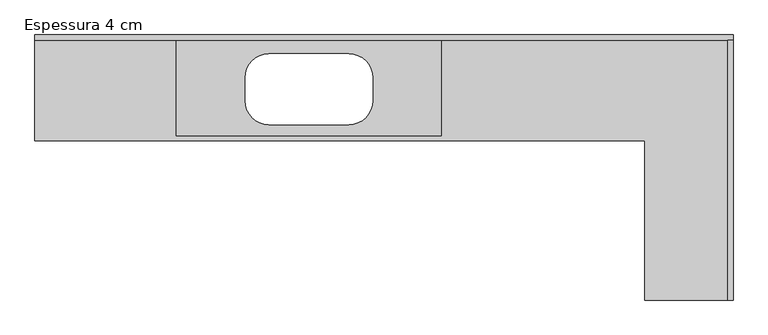
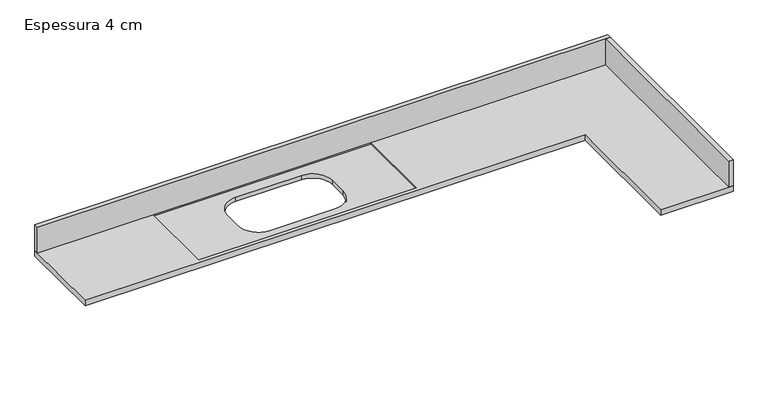
"""IFC4 building model written with IfcOpenShell, lengths in millimetres: furniture geometry, CC_BANCADA-COZINHA_EM-L_CUBA-DUPLA : Espessura 4 cm."""

import ifcopenshell
import ifcopenshell.guid

model = None  # the IFC model being written
_history = None  # IfcOwnerHistory: only IFC2X3 demands one
_inside = {}  # id of a spatial element -> (the spatial element, [elements in it])
_under = {}  # id of a project, library or spatial element -> (it, [spatial elements below it])
_declared = {}  # id of a project -> (the project, [libraries it declares])
_typed = {}  # id of a type object -> (the type object, [elements of that type])
_made_of = {}  # id of a material, layer set ... -> (it, [elements and type objects made of it])


def new_model(schema):
    """Start an empty IFC model of exactly this schema.

    Asked for "IFC4X3", IfcOpenShell would pick the latest addendum, in which some entities
    have other attributes; the version numbers below select the first issue.
    IFC2X3 requires an IfcOwnerHistory on every rooted entity: one is made here for all.
    """
    global model, _history
    if schema == "IFC4X3":
        model = ifcopenshell.file(schema_version=(4, 3, 0, 0))
    else:
        model = ifcopenshell.file(schema=schema)
    _inside.clear()
    _under.clear()
    _declared.clear()
    _typed.clear()
    _made_of.clear()
    _history = None
    if model.schema == "IFC2X3":
        org = make("IfcOrganization", Name="unknown")
        user = make(
            "IfcPersonAndOrganization",
            ThePerson=make("IfcPerson", FamilyName="unknown"),
            TheOrganization=org,
        )
        app = make(
            "IfcApplication",
            ApplicationDeveloper=org,
            Version="unknown",
            ApplicationFullName="unknown",
            ApplicationIdentifier="unknown",
        )
        _history = make(
            "IfcOwnerHistory",
            OwningUser=user,
            OwningApplication=app,
            ChangeAction="ADDED",
            CreationDate=0,
        )
    return model


def make(cls, **values):
    """One entity of the class cls with the attributes given. An attribute that is None is left unset."""
    return model.create_entity(
        cls, **{name: value for name, value in values.items() if value is not None}
    )


def rooted(cls, **values):
    """An entity with a GlobalId (a new one), such as an element, a storey or a relation."""
    return make(cls, GlobalId=ifcopenshell.guid.new(), OwnerHistory=_history, **values)


def si_unit(unit_type, name, prefix=None):
    """IfcSIUnit, for example si_unit("LENGTHUNIT", "METRE", prefix="MILLI")."""
    return make("IfcSIUnit", UnitType=unit_type, Prefix=prefix, Name=name)


def assignment(units):
    """IfcUnitAssignment: the units of a project."""
    return None if units is None else make("IfcUnitAssignment", Units=units)


def point(xyz):
    """IfcCartesianPoint."""
    return None if xyz is None else make("IfcCartesianPoint", Coordinates=xyz)


def direction(xyz):
    """IfcDirection."""
    return None if xyz is None else make("IfcDirection", DirectionRatios=xyz)


def frame(location, z_axis=None, x_axis=None):
    """IfcAxis2Placement3D, a coordinate frame: its origin and axes. An axis left out is left unset."""
    return make(
        "IfcAxis2Placement3D",
        Location=point(location),
        Axis=direction(z_axis),
        RefDirection=direction(x_axis),
    )


def origin():
    """The frame at (0, 0, 0) with its axes left unset."""
    return frame((0.0, 0.0, 0.0))


def place(relative_to, where):
    """IfcLocalPlacement: puts the frame where relative to a parent placement (None: the world)."""
    return make(
        "IfcLocalPlacement", PlacementRelTo=relative_to, RelativePlacement=where
    )


def context(
    kind, dimensions, precision=None, world=None, true_north=None, identifier=None
):
    """IfcGeometricRepresentationContext, for example the 3D "Model" context."""
    return make(
        "IfcGeometricRepresentationContext",
        ContextIdentifier=identifier,
        ContextType=kind,
        CoordinateSpaceDimension=dimensions,
        Precision=precision,
        WorldCoordinateSystem=world,
        TrueNorth=true_north,
    )


def project(units=None, contexts=None):
    """IfcProject with its units and contexts."""
    return rooted(
        "IfcProject",
        Name="project",
        RepresentationContexts=contexts,
        UnitsInContext=assignment(units),
    )


def spatial(cls, under=None, at=None, **own):
    """A site, building, storey or space (cls), placed at a placement, below another one or the project."""
    s = rooted(cls, ObjectPlacement=at, **own)
    if under is not None:
        _under.setdefault(under.id(), (under, []))[1].append(s)
    return s


def polyline(points):
    """IfcPolyline through the points."""
    return make("IfcPolyline", Points=[point(p) for p in points])


def circle_curve(where, radius):
    """IfcCircle in the frame where."""
    return make("IfcCircle", Position=where, Radius=radius)


def outline(outer, holes=None, kind="AREA"):
    """IfcArbitraryClosedProfileDef: a profile drawn as a closed curve; with holes, ...WithVoids."""
    if holes is None:
        return make("IfcArbitraryClosedProfileDef", ProfileType=kind, OuterCurve=outer)
    return make(
        "IfcArbitraryProfileDefWithVoids",
        ProfileType=kind,
        OuterCurve=outer,
        InnerCurves=holes,
    )


def extrude(swept, where, along, depth):
    """IfcExtrudedAreaSolid: the profile swept, set in the frame where, extruded along a direction by depth."""
    return make(
        "IfcExtrudedAreaSolid",
        SweptArea=swept,
        Position=where,
        ExtrudedDirection=direction(along),
        Depth=depth,
    )


def shape(context_of_items, identifier, shape_type, items):
    """IfcShapeRepresentation: the items that make up one representation, for example the "Body"."""
    return make(
        "IfcShapeRepresentation",
        ContextOfItems=context_of_items,
        RepresentationIdentifier=identifier,
        RepresentationType=shape_type,
        Items=items,
    )


def source(mapping_origin, context_of_items, identifier, shape_type, items):
    """IfcRepresentationMap: a shape defined once, which mapped items show again and again."""
    return make(
        "IfcRepresentationMap",
        MappingOrigin=mapping_origin,
        MappedRepresentation=shape(context_of_items, identifier, shape_type, items),
    )


def transform(
    local_origin,
    x_axis=None,
    y_axis=None,
    z_axis=None,
    scale=None,
    scale2=None,
    scale3=None,
    uniform=True,
):
    """IfcCartesianTransformationOperator3D, or its non-uniform kind. x_axis, y_axis, z_axis: its Axis1, 2, 3."""
    if uniform:
        return make(
            "IfcCartesianTransformationOperator3D",
            Axis1=direction(x_axis),
            Axis2=direction(y_axis),
            LocalOrigin=point(local_origin),
            Scale=scale,
            Axis3=direction(z_axis),
        )
    return make(
        "IfcCartesianTransformationOperator3DnonUniform",
        Axis1=direction(x_axis),
        Axis2=direction(y_axis),
        LocalOrigin=point(local_origin),
        Scale=scale,
        Axis3=direction(z_axis),
        Scale2=scale2,
        Scale3=scale3,
    )


def mapped(mapping_source, mapping_target):
    """IfcMappedItem: shows the shape of a source again, moved by a transform."""
    return make(
        "IfcMappedItem", MappingSource=mapping_source, MappingTarget=mapping_target
    )


def made_of(thing, what):
    """Note that an element or type object is made of a material, layer set ...; save() writes the relation."""
    if what is not None:
        _made_of.setdefault(what.id(), (what, []))[1].append(thing)
    return thing


def element(
    cls,
    number,
    at=None,
    inside=None,
    cuts=None,
    type_object=None,
    material=None,
    context=None,
    identifier="Body",
    shape_type=None,
    held_by="IfcProductDefinitionShape",
    body=None,
    shapes=None,
    **own,
):
    """One element of the class cls, such as IfcWall. Its Tag is "e" and its number.

    at: its placement. inside: the storey or other place that contains it. cuts: it is an
    opening in that element (IfcRelVoidsElement). A single representation is given by context,
    identifier, shape_type and body (its items); several are given by shapes. held_by: the class
    of the entity that holds the representations. save() writes the other relations.
    """
    e = rooted(cls, Tag="e%d" % number, ObjectPlacement=at, **own)
    if body is not None:
        shapes = [shape(context, identifier, shape_type, body)]
    if shapes is not None:
        e.Representation = make(held_by, Representations=shapes)
    if inside is not None:
        _inside.setdefault(inside.id(), (inside, []))[1].append(e)
    if cuts is not None:
        rooted(
            "IfcRelVoidsElement", RelatingBuildingElement=cuts, RelatedOpeningElement=e
        )
    if type_object is not None:
        _typed.setdefault(type_object.id(), (type_object, []))[1].append(e)
    return made_of(e, material)


def aggregate(whole, parts):
    """IfcRelAggregates: a whole, such as a stair, and the parts it consists of."""
    return rooted("IfcRelAggregates", RelatingObject=whole, RelatedObjects=parts)


def save(model, path):
    """Write the relations noted so far, then the file.

    IfcRelAggregates (storeys below a building ...), IfcRelContainedInSpatialStructure (elements
    in a storey), IfcRelDefinesByType, IfcRelAssociatesMaterial and IfcRelDeclares: one each for
    every whole, place, type object, material and project.
    """
    for whole, parts in _under.values():
        aggregate(whole, parts)
    for where, things in _inside.values():
        rooted(
            "IfcRelContainedInSpatialStructure",
            RelatedElements=things,
            RelatingStructure=where,
        )
    for kind, things in _typed.values():
        rooted("IfcRelDefinesByType", RelatedObjects=things, RelatingType=kind)
    for what, things in _made_of.values():
        rooted("IfcRelAssociatesMaterial", RelatedObjects=things, RelatingMaterial=what)
    for by, libraries in _declared.values():
        rooted("IfcRelDeclares", RelatingContext=by, RelatedDefinitions=libraries)
    model.write(path)


def plane_surface(at):
    """IfcPlane: the flat surface through the origin of the frame at, square to its z axis."""
    return make("IfcPlane", Position=at)


def revolved_surface(curve, axis_point, axis_direction):
    """IfcSurfaceOfRevolution: the curve turned about the line through axis_point along axis_direction."""
    return make(
        "IfcSurfaceOfRevolution",
        SweptCurve=make("IfcArbitraryOpenProfileDef", ProfileType="CURVE", Curve=curve),
        AxisPosition=make("IfcAxis1Placement", Location=point(axis_point), Axis=direction(axis_direction)),
    )


def advanced_brep(points, edges, surfaces, faces):
    """IfcAdvancedBrep: a solid bounded by faces that lie on surfaces and meet in shared edges.

    An edge is (start, end): straight between two places in points (the first is 0);
    or (start, end, curve); or (start, end, curve, False) where it runs against its curve.
    A face is (place in surfaces, loops), or (place, loops, False) where it looks against
    its surface's normal. A loop lists edges by number (the first is 1), with a minus sign
    where the edge is run from its end to its start. The first loop is the outer one.
    """
    corners = [point(p) for p in points]
    vertices = [make("IfcVertexPoint", VertexGeometry=c) for c in corners]
    made = []
    for start, end, *more in edges:
        made.append(
            make(
                "IfcEdgeCurve",
                EdgeStart=vertices[start],
                EdgeEnd=vertices[end],
                EdgeGeometry=more[0] if more else make("IfcPolyline", Points=[corners[start], corners[end]]),
                SameSense=more[1] if len(more) > 1 else True,
            )
        )
    hull = []
    for where, loops, *sense in faces:
        bounds = []
        for j, loop in enumerate(loops):
            ring = [make("IfcOrientedEdge", EdgeElement=made[abs(k) - 1], Orientation=k > 0) for k in loop]
            bounds.append(
                make(
                    "IfcFaceOuterBound" if j == 0 else "IfcFaceBound",
                    Bound=make("IfcEdgeLoop", EdgeList=ring),
                    Orientation=True,
                )
            )
        hull.append(make("IfcAdvancedFace", Bounds=bounds, FaceSurface=surfaces[where], SameSense=sense[0] if sense else True))
    return make("IfcAdvancedBrep", Outer=make("IfcClosedShell", CfsFaces=hull))


def espessura_4_cm_f782d00c(model_context):
    return source(origin(), model_context, "Body", "SolidModel", [
        extrude(outline(polyline([(-30.0, -30.0), (0.0, -30.0), (0.0, -1500.0), (-30.0, -1500.0), (-30.0, -30.0)])), frame((0.0, 0.0, 900.0), z_axis=(0.0, 0.0, 1.0), x_axis=(1.0, 0.0, 0.0)), (0.0, 0.0, 1.0), 190.0),
        extrude(outline(polyline([(-3950.0, -30.0), (-3950.0, 0.0), (0.0, 0.0), (0.0, -30.0), (-3950.0, -30.0)])), frame((0.0, 0.0, 900.0), z_axis=(0.0, 0.0, 1.0), x_axis=(1.0, 0.0, 0.0)), (0.0, 0.0, 1.0), 190.0),
        advanced_brep(
        [(-500.0, -600.0, 860.0), (-3950.0, -600.0, 860.0), (-3950.0, 0.0, 860.0), (0.0, 0.0, 860.0), (0.0, -1500.0, 860.0), (-500.0, -1500.0, 860.0), (-2626.0, -107.0, 860.0), (-2761.0, -242.0, 860.0), (-2761.0, -372.0, 860.0), (-2626.0, -507.0, 860.0), (-2174.0, -507.0, 860.0), (-2039.0, -372.0, 860.0), (-2039.0, -242.0, 860.0), (-2174.0, -107.0, 860.0), (-500.0, -600.0, 900.0), (-500.0, -1500.0, 900.0), (0.0, -1500.0, 900.0), (0.0, 0.0, 900.0), (-3950.0, 0.0, 900.0), (-3950.0, -600.0, 900.0), (-1650.0, -30.0, 900.0), (-1650.0, -570.0, 900.0), (-3150.0, -570.0, 900.0), (-3150.0, -30.0, 900.0), (-2174.0, -107.0, 890.0), (-2626.0, -107.0, 890.0), (-2039.0, -242.0, 890.0), (-2039.0, -372.0, 890.0), (-2174.0, -507.0, 890.0), (-2626.0, -507.0, 890.0), (-2761.0, -372.0, 890.0), (-2761.0, -242.0, 890.0), (-1650.0, -570.0, 890.0), (-1650.0, -30.0, 890.0), (-3150.0, -30.0, 890.0), (-3150.0, -570.0, 890.0)],
        [
            (0, 1),
            (1, 2),
            (2, 3),
            (3, 4),
            (4, 5),
            (5, 0),
            (6, 7, circle_curve(frame((-2626.0, -242.0, 860.0), z_axis=(0.0, 0.0, 1.0), x_axis=(-1.0, 0.0, 0.0)), 135.0)),
            (7, 8),
            (8, 9, circle_curve(frame((-2626.0, -372.0, 860.0), z_axis=(0.0, 0.0, 1.0), x_axis=(-1.0, 0.0, 0.0)), 135.0)),
            (9, 10),
            (10, 11, circle_curve(frame((-2174.0, -372.0, 860.0), z_axis=(0.0, 0.0, 1.0), x_axis=(-1.0, 0.0, 0.0)), 135.0)),
            (11, 12),
            (12, 13, circle_curve(frame((-2174.0, -242.0, 860.0), z_axis=(0.0, 0.0, 1.0), x_axis=(-1.0, 0.0, 0.0)), 135.0)),
            (13, 6),
            (14, 15),
            (15, 16),
            (16, 17),
            (17, 18),
            (18, 19),
            (19, 14),
            (20, 21),
            (21, 22),
            (22, 23),
            (23, 20),
            (5, 15),
            (14, 0),
            (4, 16),
            (3, 17),
            (2, 18),
            (1, 19),
            (13, 24),
            (24, 25),
            (25, 6),
            (12, 26),
            (26, 24, circle_curve(frame((-2174.0, -242.0, 890.0), z_axis=(0.0, 0.0, 1.0), x_axis=(-1.0, 0.0, 0.0)), 135.0)),
            (11, 27),
            (27, 26),
            (10, 28),
            (28, 27, circle_curve(frame((-2174.0, -372.0, 890.0), z_axis=(0.0, 0.0, 1.0), x_axis=(-1.0, 0.0, 0.0)), 135.0)),
            (9, 29),
            (29, 28),
            (8, 30),
            (30, 29, circle_curve(frame((-2626.0, -372.0, 890.0), z_axis=(0.0, 0.0, 1.0), x_axis=(-1.0, 0.0, 0.0)), 135.0)),
            (7, 31),
            (31, 30),
            (25, 31, circle_curve(frame((-2626.0, -242.0, 890.0), z_axis=(0.0, 0.0, 1.0), x_axis=(-1.0, 0.0, 0.0)), 135.0)),
            (32, 33),
            (33, 34),
            (34, 35),
            (35, 32),
            (32, 21),
            (20, 33),
            (23, 34),
            (22, 35),
        ],
        [
            plane_surface(frame((-500.0, -600.0, 860.0), z_axis=(0.0, 0.0, -1.0), x_axis=(0.0, 1.0, 0.0))),
            plane_surface(frame((-500.0, -600.0, 900.0), z_axis=(0.0, 0.0, 1.0), x_axis=(0.0, -1.0, 0.0))),
            plane_surface(frame((-500.0, -600.0, 900.0), z_axis=(-1.0, 0.0, 0.0), x_axis=(0.0, 0.0, -1.0))),
            plane_surface(frame((-500.0, -1500.0, 900.0), z_axis=(0.0, -1.0, 0.0), x_axis=(0.0, 0.0, -1.0))),
            plane_surface(frame((0.0, -1500.0, 900.0), z_axis=(1.0, 0.0, 0.0), x_axis=(0.0, 0.0, -1.0))),
            plane_surface(frame((0.0, 0.0, 900.0), z_axis=(0.0, 1.0, 0.0), x_axis=(0.0, 0.0, -1.0))),
            plane_surface(frame((-3950.0, 0.0, 900.0), z_axis=(-1.0, 0.0, 0.0), x_axis=(0.0, 0.0, -1.0))),
            plane_surface(frame((-3950.0, -600.0, 900.0), z_axis=(0.0, -1.0, 0.0), x_axis=(0.0, 0.0, -1.0))),
            plane_surface(frame((-2626.0, -107.0, 900.0), z_axis=(0.0, -1.0, 0.0), x_axis=(0.0, 0.0, -1.0))),
            revolved_surface(polyline([(-2309.0, -242.0, 860.0), (-2309.0, -242.0, 890.0)]), (-2174.0, -242.0, 890.0), (0.0, 0.0, -1.0)),
            plane_surface(frame((-2039.0, -242.0, 900.0), z_axis=(-1.0, 0.0, 0.0), x_axis=(0.0, 0.0, -1.0))),
            revolved_surface(polyline([(-2309.0, -372.0, 860.0), (-2309.0, -372.0, 890.0)]), (-2174.0, -372.0, 890.0), (0.0, 0.0, -1.0)),
            plane_surface(frame((-2174.0, -507.0, 900.0), z_axis=(0.0, 1.0, 0.0), x_axis=(0.0, 0.0, -1.0))),
            revolved_surface(polyline([(-2761.0, -372.0, 860.0), (-2761.0, -372.0, 890.0)]), (-2626.0, -372.0, 890.0), (0.0, 0.0, -1.0)),
            plane_surface(frame((-2761.0, -372.0, 900.0), z_axis=(1.0, 0.0, 0.0), x_axis=(0.0, 0.0, -1.0))),
            revolved_surface(polyline([(-2761.0, -242.0, 860.0), (-2761.0, -242.0, 890.0)]), (-2626.0, -242.0, 890.0), (0.0, 0.0, -1.0)),
            plane_surface(frame((-1650.0, -30.0, 890.0), z_axis=(0.0, 0.0, 1.0), x_axis=(0.0, -1.0, 0.0))),
            plane_surface(frame((-1650.0, -570.0, 940.0), z_axis=(-1.0, 0.0, 0.0), x_axis=(0.0, 0.0, -1.0))),
            plane_surface(frame((-1650.0, -30.0, 940.0), z_axis=(0.0, -1.0, 0.0), x_axis=(0.0, 0.0, -1.0))),
            plane_surface(frame((-3150.0, -30.0, 940.0), z_axis=(1.0, 0.0, 0.0), x_axis=(0.0, 0.0, -1.0))),
            plane_surface(frame((-3150.0, -570.0, 940.0), z_axis=(0.0, 1.0, 0.0), x_axis=(0.0, 0.0, -1.0))),
        ],
        [
            (0, [[1, 2, 3, 4, 5, 6], [7, 8, 9, 10, 11, 12, 13, 14]]),
            (1, [[15, 16, 17, 18, 19, 20], [21, 22, 23, 24]]),
            (2, [[-6, 25, -15, 26]]),
            (3, [[-5, 27, -16, -25]]),
            (4, [[-4, 28, -17, -27]]),
            (5, [[-3, 29, -18, -28]]),
            (6, [[-2, 30, -19, -29]]),
            (7, [[-1, -26, -20, -30]]),
            (8, [[-14, 31, 32, 33]]),
            (9, [[-13, 34, 35, -31]]),
            (10, [[-12, 36, 37, -34]]),
            (11, [[-11, 38, 39, -36]]),
            (12, [[-10, 40, 41, -38]]),
            (13, [[-9, 42, 43, -40]]),
            (14, [[-8, 44, 45, -42]]),
            (15, [[-7, -33, 46, -44]]),
            (16, [[47, 48, 49, 50], [-32, -35, -37, -39, -41, -43, -45, -46]]),
            (17, [[-47, 51, -21, 52]]),
            (18, [[-48, -52, -24, 53]]),
            (19, [[-49, -53, -23, 54]]),
            (20, [[-50, -54, -22, -51]]),
        ],
    ),
    ])


if __name__ == "__main__":
    model = new_model("IFC4")
    model_context = context("Model", 3, world=origin())
    ifc_project = project(units=[si_unit("LENGTHUNIT", "METRE", prefix="MILLI")], contexts=[model_context])
    site = spatial("IfcSite", under=ifc_project)
    building = spatial("IfcBuilding", under=site)
    placement = place(None, origin())
    espessura_4_cm_shape = espessura_4_cm_f782d00c(model_context)
    element("IfcFurniture", 1, ObjectType="CC_BANCADA-COZINHA_EM-L_CUBA-DUPLA : Espessura 4 cm", at=placement, inside=building, context=model_context, shape_type="MappedRepresentation", body=[
        mapped(espessura_4_cm_shape, transform((0.0, 0.0, 0.0), x_axis=(1.0, 0.0, 0.0), y_axis=(0.0, 1.0, 0.0), z_axis=(0.0, 0.0, 1.0))),
    ])
    save(model, "model.ifc")

# Revit data of these elements
# Type "CC_BANCADA-COZINHA_EM-L_CUBA-DUPLA : Espessura 4 cm"
#   Uso HS [instance default] = ""
#   Offset esq área molhada [instance default] = 0.80 m
#   Largura área molhada [instance default] = 1.50 m
#   Largura principal [instance default] = 0.60 m
#   Largura da extensão [instance default] = 0.50 m
#   Espessura total da bancada [instance default] = 0.04 m
#   Espessura do frontão [instance default] = 0.03 m
#   Dist. cuba - borda [instance default] = 0.07 m
#   Compr. total principal [instance default] = 3.95 m
#   Compr. principal [instance default] = 3.45 m
#   Compr. total extensão [instance default] = 1.50 m
#   Compr. extensão [instance default] = 0.90 m
#   Altura do rebaixo da área molhada [instance default] = 0.01 m
#   Altura do frontão [instance default] = 0.20 m
#   Altura da bancada [instance default] = 0.90 m
#   Frontão fundos principal [instance default] = yes
#   Frontão fundos extensão [instance default] = yes
#   Frontão esquerdo principal [instance default] = yes
#   Frontão direito extensão [instance default] = yes
#   Material da bancada [instance default] = none
# Element 1 (IfcFurniture, "CC_BANCADA-COZINHA_EM-L_CUBA-DUPLA : Espessura 4 cm")
#   Uso HS = "COZINHA"
#   Frontão esquerdo principal = no
#   Frontão direito extensão = no
#   Material da bancada = .GRANITO_BRANCO_ITAUNAS
#   Materials on its faces: ".GRANITO_BRANCO_ITAUNAS"
# Materials
#   ".GRANITO_BRANCO_ITAUNAS": class ".CC_PEDRA REVEST.", colour RGB 202 195 174, transparency 0, Description = "Revestimento em granito", Cost = 0
